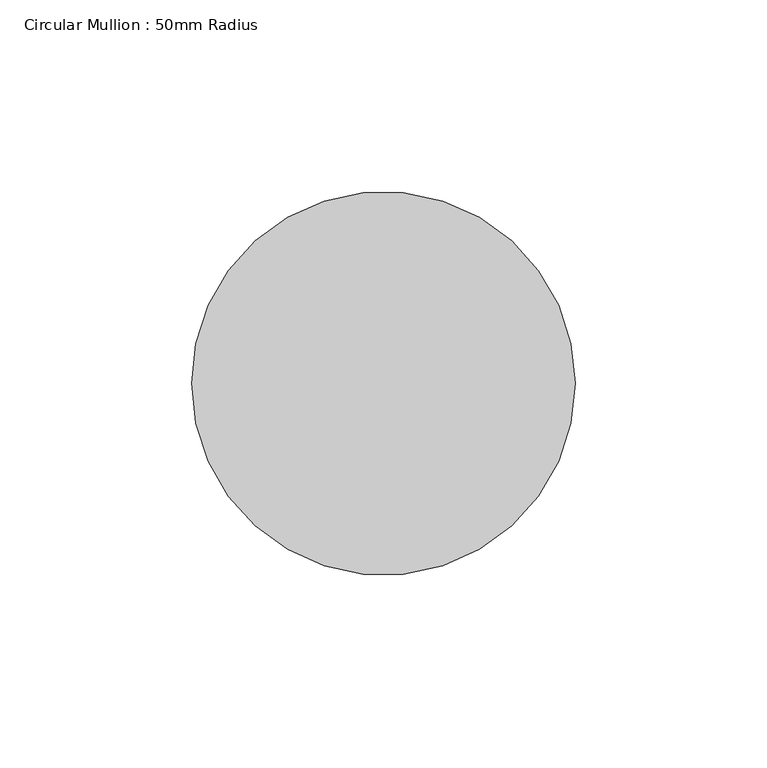
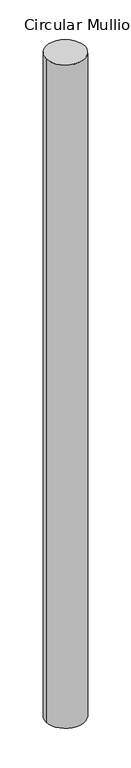
"""IFC4 building model written with IfcOpenShell, lengths in millimetres: member geometry, Circular Mullion : 50mm Radius."""

from ifc_helpers import new_model, si_unit, point, frame, origin, origin_2d, place, context, project, spatial, circle_curve, trimmed, segment, composite_curve, outline, extrude, source, transform, mapped, element, save


def circular_mullion_50mm_radius_744b49a1(model_context):
    return source(origin(), model_context, "Body", "SweptSolid", [
        extrude(outline(composite_curve([segment(trimmed(circle_curve(origin_2d(), 50.0), [point((50.0, 0.0))], [point((-50.0, 0.0))], False, "CARTESIAN"), True, "CONTINUOUS"), segment(trimmed(circle_curve(origin_2d(), 50.0), [point((-50.0, 0.0))], [point((50.0, 0.0))], False, "CARTESIAN"), True, "CONTINUOUS")], self_intersect=False)), frame((0.0, 0.0, -1817.7522087), z_axis=(0.0, 0.0, 1.0), x_axis=(1.0, 0.0, 0.0)), (0.0, 0.0, 1.0), 1817.7522087),
    ])


if __name__ == "__main__":
    model = new_model("IFC4")
    model_context = context("Model", 3, world=origin())
    ifc_project = project(units=[si_unit("LENGTHUNIT", "METRE", prefix="MILLI")], contexts=[model_context])
    site = spatial("IfcSite", under=ifc_project)
    building = spatial("IfcBuilding", under=site)
    placement = place(None, origin())
    circular_mullion_50mm_radius_shape = circular_mullion_50mm_radius_744b49a1(model_context)
    element("IfcMember", 1, ObjectType="Circular Mullion : 50mm Radius", at=placement, inside=building, context=model_context, shape_type="MappedRepresentation", body=[
        mapped(circular_mullion_50mm_radius_shape, transform((0.0, 0.0, 0.0), x_axis=(1.0, 0.0, 0.0), y_axis=(0.0, 1.0, 0.0), z_axis=(0.0, 0.0, 1.0))),
    ])
    save(model, "model.ifc")

# Revit data of these elements
# Type "Circular Mullion : 50mm Radius"
#   built-in parameter 1007350 = 0.164042 (stored number, unit not read)
# Element 1 (IfcMember, "Circular Mullion : 50mm Radius")
#   Materials on its faces: "Aluminium"
# Materials
#   "Aluminium": class "Metal", colour RGB 247 247 247, transparency 0, Description = "Aluminium 6061", Cost = 0
